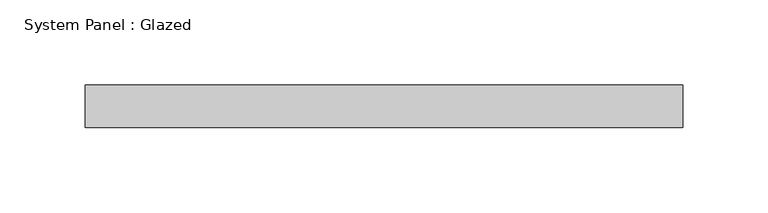
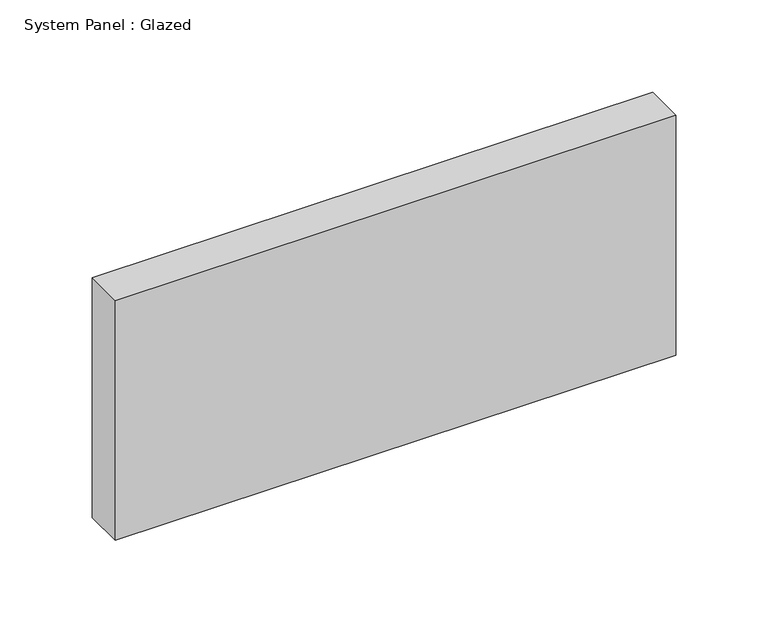
"""IFC4 building model written with IfcOpenShell, lengths in millimetres: plate geometry, System Panel : Glazed."""

from ifc_helpers import new_model, si_unit, origin, origin_with_axes, place, context, project, spatial, polyline, outline, extrude, source, transform, mapped, element, save


def system_panel_glazed_40e85cb7(model_context):
    return source(origin(), model_context, "Body", "SweptSolid", [
        extrude(outline(polyline([(175.0, 24.5), (-175.0, 24.5), (-175.0, 49.5), (175.0, 49.5), (175.0, 24.5)])), origin_with_axes(), (0.0, 0.0, 1.0), 158.3333333),
    ])


if __name__ == "__main__":
    model = new_model("IFC4")
    model_context = context("Model", 3, world=origin())
    ifc_project = project(units=[si_unit("LENGTHUNIT", "METRE", prefix="MILLI")], contexts=[model_context])
    site = spatial("IfcSite", under=ifc_project)
    building = spatial("IfcBuilding", under=site)
    placement = place(None, origin())
    system_panel_glazed_shape = system_panel_glazed_40e85cb7(model_context)
    element("IfcPlate", 1, ObjectType="System Panel : Glazed", at=placement, inside=building, context=model_context, shape_type="MappedRepresentation", body=[
        mapped(system_panel_glazed_shape, transform((0.0, 0.0, 0.0), x_axis=(1.0, 0.0, 0.0), y_axis=(0.0, 1.0, 0.0), z_axis=(0.0, 0.0, 1.0))),
    ])
    save(model, "model.ifc")

# Revit data of these elements
# Element 1 (IfcPlate, "System Panel : Glazed")
#   Materials on its faces: "Glass"
# Materials
#   "Glass": class "Glass", colour RGB 218 227 224, transparency 0.85, Description = "Soda Lime Glass", Cost = 0
